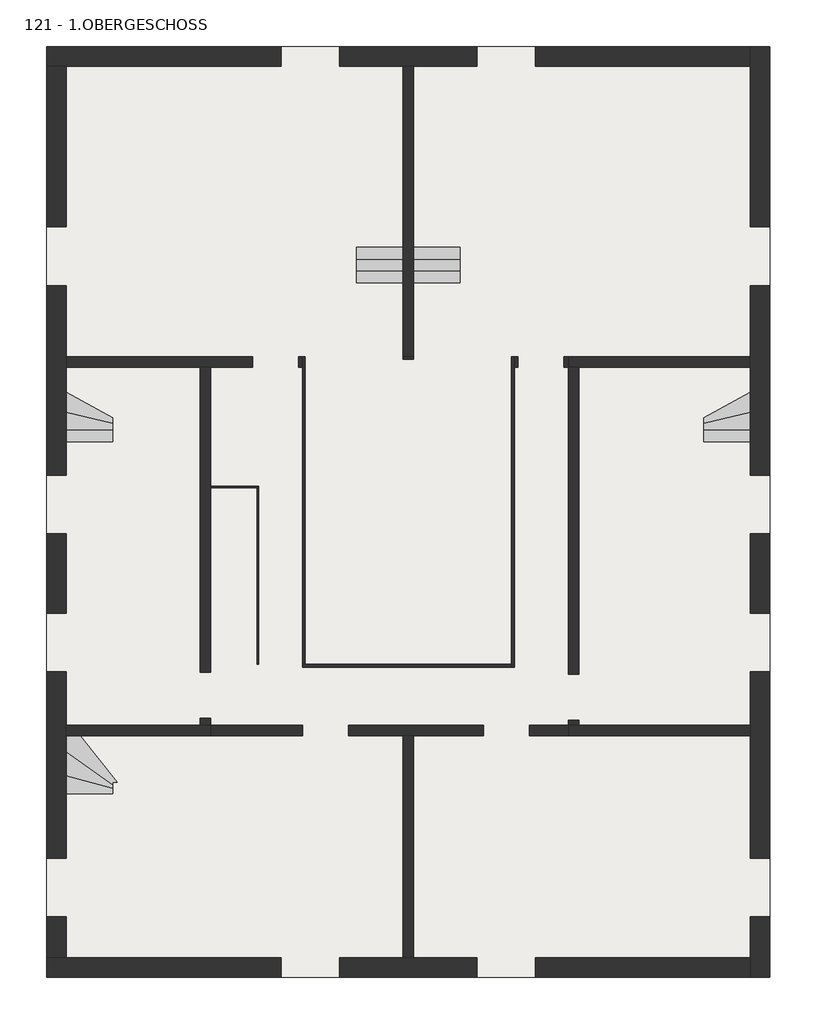
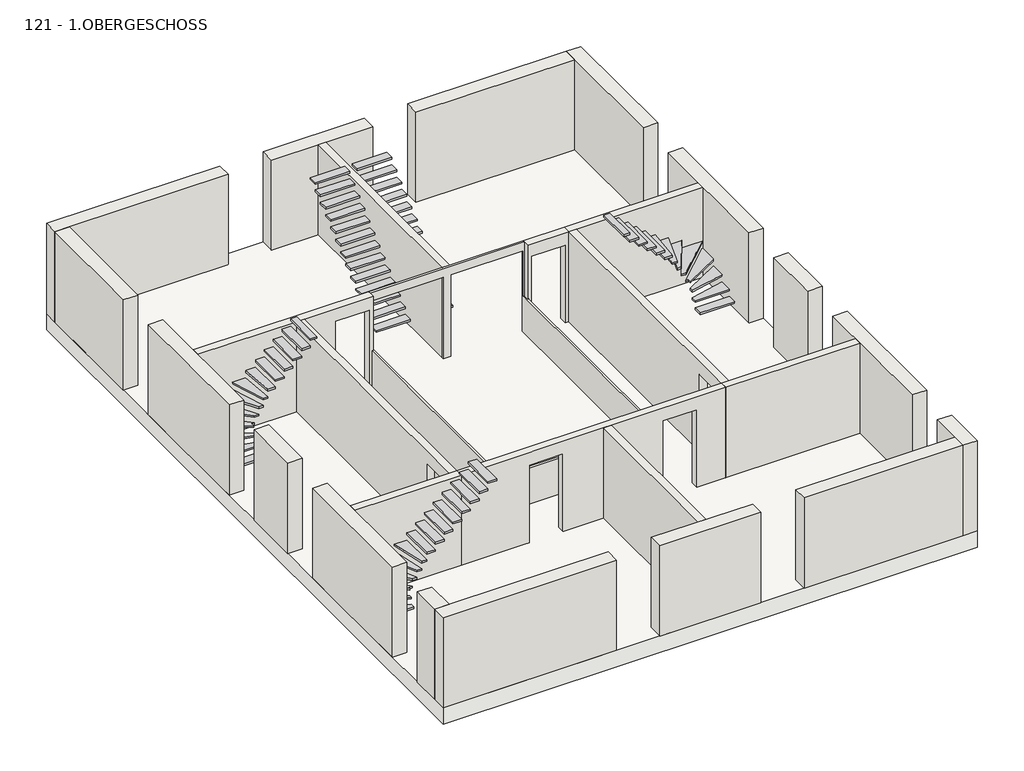
# One storey: 20 walls, 10 stairs, 1 slab.
"""IFC4 building model written with IfcOpenShell, lengths in millimetres."""

import ifcopenshell
import ifcopenshell.guid

model = None  # the IFC model being written
_history = None  # IfcOwnerHistory: only IFC2X3 demands one
_inside = {}  # id of a spatial element -> (the spatial element, [elements in it])
_under = {}  # id of a project, library or spatial element -> (it, [spatial elements below it])
_declared = {}  # id of a project -> (the project, [libraries it declares])
_typed = {}  # id of a type object -> (the type object, [elements of that type])
_made_of = {}  # id of a material, layer set ... -> (it, [elements and type objects made of it])


def new_model(schema):
    """Start an empty IFC model of exactly this schema.

    Asked for "IFC4X3", IfcOpenShell would pick the latest addendum, in which some entities
    have other attributes; the version numbers below select the first issue.
    IFC2X3 requires an IfcOwnerHistory on every rooted entity: one is made here for all.
    """
    global model, _history
    if schema == "IFC4X3":
        model = ifcopenshell.file(schema_version=(4, 3, 0, 0))
    else:
        model = ifcopenshell.file(schema=schema)
    _inside.clear()
    _under.clear()
    _declared.clear()
    _typed.clear()
    _made_of.clear()
    _history = None
    if model.schema == "IFC2X3":
        org = make("IfcOrganization", Name="unknown")
        user = make(
            "IfcPersonAndOrganization",
            ThePerson=make("IfcPerson", FamilyName="unknown"),
            TheOrganization=org,
        )
        app = make(
            "IfcApplication",
            ApplicationDeveloper=org,
            Version="unknown",
            ApplicationFullName="unknown",
            ApplicationIdentifier="unknown",
        )
        _history = make(
            "IfcOwnerHistory",
            OwningUser=user,
            OwningApplication=app,
            ChangeAction="ADDED",
            CreationDate=0,
        )
    return model


def make(cls, **values):
    """One entity of the class cls with the attributes given. An attribute that is None is left unset."""
    return model.create_entity(
        cls, **{name: value for name, value in values.items() if value is not None}
    )


def rooted(cls, **values):
    """An entity with a GlobalId (a new one), such as an element, a storey or a relation."""
    return make(cls, GlobalId=ifcopenshell.guid.new(), OwnerHistory=_history, **values)


def si_unit(unit_type, name, prefix=None):
    """IfcSIUnit, for example si_unit("LENGTHUNIT", "METRE", prefix="MILLI")."""
    return make("IfcSIUnit", UnitType=unit_type, Prefix=prefix, Name=name)


def assignment(units):
    """IfcUnitAssignment: the units of a project."""
    return None if units is None else make("IfcUnitAssignment", Units=units)


def point(xyz):
    """IfcCartesianPoint."""
    return None if xyz is None else make("IfcCartesianPoint", Coordinates=xyz)


def direction(xyz):
    """IfcDirection."""
    return None if xyz is None else make("IfcDirection", DirectionRatios=xyz)


def frame(location, z_axis=None, x_axis=None):
    """IfcAxis2Placement3D, a coordinate frame: its origin and axes. An axis left out is left unset."""
    return make(
        "IfcAxis2Placement3D",
        Location=point(location),
        Axis=direction(z_axis),
        RefDirection=direction(x_axis),
    )


def origin():
    """The frame at (0, 0, 0) with its axes left unset."""
    return frame((0.0, 0.0, 0.0))


def place(relative_to, where):
    """IfcLocalPlacement: puts the frame where relative to a parent placement (None: the world)."""
    return make(
        "IfcLocalPlacement", PlacementRelTo=relative_to, RelativePlacement=where
    )


def context(
    kind, dimensions, precision=None, world=None, true_north=None, identifier=None
):
    """IfcGeometricRepresentationContext, for example the 3D "Model" context."""
    return make(
        "IfcGeometricRepresentationContext",
        ContextIdentifier=identifier,
        ContextType=kind,
        CoordinateSpaceDimension=dimensions,
        Precision=precision,
        WorldCoordinateSystem=world,
        TrueNorth=true_north,
    )


def project(units=None, contexts=None):
    """IfcProject with its units and contexts."""
    return rooted(
        "IfcProject",
        Name="project",
        RepresentationContexts=contexts,
        UnitsInContext=assignment(units),
    )


def spatial(cls, under=None, at=None, **own):
    """A site, building, storey or space (cls), placed at a placement, below another one or the project."""
    s = rooted(cls, ObjectPlacement=at, **own)
    if under is not None:
        _under.setdefault(under.id(), (under, []))[1].append(s)
    return s


def polyline(points):
    """IfcPolyline through the points."""
    return make("IfcPolyline", Points=[point(p) for p in points])


def outline(outer, holes=None, kind="AREA"):
    """IfcArbitraryClosedProfileDef: a profile drawn as a closed curve; with holes, ...WithVoids."""
    if holes is None:
        return make("IfcArbitraryClosedProfileDef", ProfileType=kind, OuterCurve=outer)
    return make(
        "IfcArbitraryProfileDefWithVoids",
        ProfileType=kind,
        OuterCurve=outer,
        InnerCurves=holes,
    )


def extrude(swept, where, along, depth):
    """IfcExtrudedAreaSolid: the profile swept, set in the frame where, extruded along a direction by depth."""
    return make(
        "IfcExtrudedAreaSolid",
        SweptArea=swept,
        Position=where,
        ExtrudedDirection=direction(along),
        Depth=depth,
    )


def faces_of(points, faces, orient=None, outer=None):
    """IfcFace entities. A face is a list of loops; a loop is a list of indices into points, from 0.

    orient and outer hold one flag for each loop. By default every Orientation is true, the
    first loop of a face is its IfcFaceOuterBound and the others are IfcFaceBound.
    """
    made = []
    for i, loops in enumerate(faces):
        bounds = []
        for j, loop in enumerate(loops):
            is_outer = j == 0 if outer is None else outer[i][j]
            bounds.append(
                make(
                    "IfcFaceOuterBound" if is_outer else "IfcFaceBound",
                    Bound=make("IfcPolyLoop", Polygon=[points[k] for k in loop]),
                    Orientation=True if orient is None else orient[i][j],
                )
            )
        made.append(make("IfcFace", Bounds=bounds))
    return made


def faceted_brep(points, faces, orient=None, outer=None, voids=None):
    """IfcFacetedBrep: a solid bounded by flat faces; with voids (closed shells), ...WithVoids."""
    shared = [point(p) for p in points]
    hull = make("IfcClosedShell", CfsFaces=faces_of(shared, faces, orient, outer))
    if voids is None:
        return make("IfcFacetedBrep", Outer=hull)
    return make(
        "IfcFacetedBrepWithVoids",
        Outer=hull,
        Voids=[
            make(cls, CfsFaces=faces_of(shared, fs, o, b)) for cls, fs, o, b in voids
        ],
    )


def shape(context_of_items, identifier, shape_type, items):
    """IfcShapeRepresentation: the items that make up one representation, for example the "Body"."""
    return make(
        "IfcShapeRepresentation",
        ContextOfItems=context_of_items,
        RepresentationIdentifier=identifier,
        RepresentationType=shape_type,
        Items=items,
    )


def source(mapping_origin, context_of_items, identifier, shape_type, items):
    """IfcRepresentationMap: a shape defined once, which mapped items show again and again."""
    return make(
        "IfcRepresentationMap",
        MappingOrigin=mapping_origin,
        MappedRepresentation=shape(context_of_items, identifier, shape_type, items),
    )


def transform(
    local_origin,
    x_axis=None,
    y_axis=None,
    z_axis=None,
    scale=None,
    scale2=None,
    scale3=None,
    uniform=True,
):
    """IfcCartesianTransformationOperator3D, or its non-uniform kind. x_axis, y_axis, z_axis: its Axis1, 2, 3."""
    if uniform:
        return make(
            "IfcCartesianTransformationOperator3D",
            Axis1=direction(x_axis),
            Axis2=direction(y_axis),
            LocalOrigin=point(local_origin),
            Scale=scale,
            Axis3=direction(z_axis),
        )
    return make(
        "IfcCartesianTransformationOperator3DnonUniform",
        Axis1=direction(x_axis),
        Axis2=direction(y_axis),
        LocalOrigin=point(local_origin),
        Scale=scale,
        Axis3=direction(z_axis),
        Scale2=scale2,
        Scale3=scale3,
    )


def mapped(mapping_source, mapping_target):
    """IfcMappedItem: shows the shape of a source again, moved by a transform."""
    return make(
        "IfcMappedItem", MappingSource=mapping_source, MappingTarget=mapping_target
    )


def made_of(thing, what):
    """Note that an element or type object is made of a material, layer set ...; save() writes the relation."""
    if what is not None:
        _made_of.setdefault(what.id(), (what, []))[1].append(thing)
    return thing


def element(
    cls,
    number,
    at=None,
    inside=None,
    cuts=None,
    type_object=None,
    material=None,
    context=None,
    identifier="Body",
    shape_type=None,
    held_by="IfcProductDefinitionShape",
    body=None,
    shapes=None,
    **own,
):
    """One element of the class cls, such as IfcWall. Its Tag is "e" and its number.

    at: its placement. inside: the storey or other place that contains it. cuts: it is an
    opening in that element (IfcRelVoidsElement). A single representation is given by context,
    identifier, shape_type and body (its items); several are given by shapes. held_by: the class
    of the entity that holds the representations. save() writes the other relations.
    """
    e = rooted(cls, Tag="e%d" % number, ObjectPlacement=at, **own)
    if body is not None:
        shapes = [shape(context, identifier, shape_type, body)]
    if shapes is not None:
        e.Representation = make(held_by, Representations=shapes)
    if inside is not None:
        _inside.setdefault(inside.id(), (inside, []))[1].append(e)
    if cuts is not None:
        rooted(
            "IfcRelVoidsElement", RelatingBuildingElement=cuts, RelatedOpeningElement=e
        )
    if type_object is not None:
        _typed.setdefault(type_object.id(), (type_object, []))[1].append(e)
    return made_of(e, material)


def aggregate(whole, parts):
    """IfcRelAggregates: a whole, such as a stair, and the parts it consists of."""
    return rooted("IfcRelAggregates", RelatingObject=whole, RelatedObjects=parts)


def save(model, path):
    """Write the relations noted so far, then the file.

    IfcRelAggregates (storeys below a building ...), IfcRelContainedInSpatialStructure (elements
    in a storey), IfcRelDefinesByType, IfcRelAssociatesMaterial and IfcRelDeclares: one each for
    every whole, place, type object, material and project.
    """
    for whole, parts in _under.values():
        aggregate(whole, parts)
    for where, things in _inside.values():
        rooted(
            "IfcRelContainedInSpatialStructure",
            RelatedElements=things,
            RelatingStructure=where,
        )
    for kind, things in _typed.values():
        rooted("IfcRelDefinesByType", RelatedObjects=things, RelatingType=kind)
    for what, things in _made_of.values():
        rooted("IfcRelAssociatesMaterial", RelatedObjects=things, RelatingMaterial=what)
    for by, libraries in _declared.values():
        rooted("IfcRelDeclares", RelatingContext=by, RelatedDefinitions=libraries)
    model.write(path)


def slab_91406d58(model_context):
    return source(origin(), model_context, "Body", "SweptSolid", [
        extrude(outline(polyline([(15500.0, 19550.0), (15500.0, 1547.1380981), (1500.0, 1547.1380981), (1500.0, 19550.0), (15500.0, 19550.0)])), frame((0.0, 0.0, 2880.0), z_axis=(0.0, 0.0, 1.0), x_axis=(1.0, 0.0, 0.0)), (0.0, 0.0, 1.0), 450.0),
    ])


def stair_92ba3d55(model_context):
    return source(origin(), model_context, "Body", "SweptSolid", [
        extrude(outline(polyline([(160077.7593015, 32139.1812131), (160077.7593015, 32029.7962965), (159177.7593015, 32029.7962965), (159177.7593015, 32381.5903923), (160077.7593015, 32139.1812131)])), frame((0.0, 0.0, 3480.0), z_axis=(0.0, 0.0, 1.0), x_axis=(1.0, 0.0, 0.0)), (0.0, 0.0, 1.0), 50.0),
        extrude(outline(polyline([(160077.7593015, 32208.6851854), (160077.7593015, 32139.1812131), (159177.7593015, 32381.5903923), (159177.7593015, 32851.1265298), (160077.7593015, 32208.6851854)])), frame((0.0, 0.0, 3680.0), z_axis=(0.0, 0.0, 1.0), x_axis=(1.0, 0.0, 0.0)), (0.0, 0.0, 1.0), 50.0),
        extrude(outline(polyline([(159450.38828, 33159.7962965), (160164.4298971, 32259.7962965), (160077.7593015, 32259.7962965), (160077.7593015, 32208.6851854), (159177.7593015, 32851.1265298), (159177.7593015, 33159.7962965), (159450.38828, 33159.7962965)])), frame((0.0, 0.0, 3880.0), z_axis=(0.0, 0.0, 1.0), x_axis=(1.0, 0.0, 0.0)), (0.0, 0.0, 1.0), 50.0),
        extrude(outline(polyline([(160285.4396784, 32259.7962965), (160164.4298971, 32259.7962965), (159450.38828, 33159.7962965), (159877.5404106, 33159.7962965), (160285.4396784, 32259.7962965)])), frame((0.0, 0.0, 4080.0), z_axis=(0.0, 0.0, 1.0), x_axis=(1.0, 0.0, 0.0)), (0.0, 0.0, 1.0), 50.0),
        extrude(outline(polyline([(160412.2916695, 32259.7962965), (160285.4396784, 32259.7962965), (159877.5404106, 33159.7962965), (160212.4306066, 33159.7962965), (160412.2916695, 32259.7962965)])), frame((0.0, 0.0, 4280.0), z_axis=(0.0, 0.0, 1.0), x_axis=(1.0, 0.0, 0.0)), (0.0, 0.0, 1.0), 50.0),
        extrude(outline(polyline([(160546.5910216, 32259.7962965), (160412.2916695, 32259.7962965), (160212.4306066, 33159.7962965), (160538.1312545, 33159.7962965), (160546.5910216, 32259.7962965)])), frame((0.0, 0.0, 4480.0), z_axis=(0.0, 0.0, 1.0), x_axis=(1.0, 0.0, 0.0)), (0.0, 0.0, 1.0), 50.0),
        extrude(outline(polyline([(160772.3611381, 32259.7962965), (160546.5910216, 32259.7962965), (160538.1312545, 33159.7962965), (160772.3611381, 33159.7962965), (160772.3611381, 32259.7962965)])), frame((0.0, 0.0, 4680.0), z_axis=(0.0, 0.0, 1.0), x_axis=(1.0, 0.0, 0.0)), (0.0, 0.0, 1.0), 50.0),
        extrude(outline(polyline([(161002.3611381, 32259.7962965), (160772.3611381, 32259.7962965), (160772.3611381, 33159.7962965), (161002.3611381, 33159.7962965), (161002.3611381, 32259.7962965)])), frame((0.0, 0.0, 4880.0), z_axis=(0.0, 0.0, 1.0), x_axis=(1.0, 0.0, 0.0)), (0.0, 0.0, 1.0), 50.0),
        extrude(outline(polyline([(161232.3611381, 32259.7962965), (161002.3611381, 32259.7962965), (161002.3611381, 33159.7962965), (161232.3611381, 33159.7962965), (161232.3611381, 32259.7962965)])), frame((0.0, 0.0, 5080.0), z_axis=(0.0, 0.0, 1.0), x_axis=(1.0, 0.0, 0.0)), (0.0, 0.0, 1.0), 50.0),
        extrude(outline(polyline([(161462.3611381, 32259.7962965), (161232.3611381, 32259.7962965), (161232.3611381, 33159.7962965), (161462.3611381, 33159.7962965), (161462.3611381, 32259.7962965)])), frame((0.0, 0.0, 5280.0), z_axis=(0.0, 0.0, 1.0), x_axis=(1.0, 0.0, 0.0)), (0.0, 0.0, 1.0), 50.0),
        extrude(outline(polyline([(161692.3611381, 32259.7962965), (161462.3611381, 32259.7962965), (161462.3611381, 33159.7962965), (161692.3611381, 33159.7962965), (161692.3611381, 32259.7962965)])), frame((0.0, 0.0, 5480.0), z_axis=(0.0, 0.0, 1.0), x_axis=(1.0, 0.0, 0.0)), (0.0, 0.0, 1.0), 50.0),
        extrude(outline(polyline([(161922.3611381, 32259.7962965), (161692.3611381, 32259.7962965), (161692.3611381, 33159.7962965), (161922.3611381, 33159.7962965), (161922.3611381, 32259.7962965)])), frame((0.0, 0.0, 5680.0), z_axis=(0.0, 0.0, 1.0), x_axis=(1.0, 0.0, 0.0)), (0.0, 0.0, 1.0), 50.0),
        extrude(outline(polyline([(162152.3611381, 32259.7962965), (161922.3611381, 32259.7962965), (161922.3611381, 33159.7962965), (162152.3611381, 33159.7962965), (162152.3611381, 32259.7962965)])), frame((0.0, 0.0, 5880.0), z_axis=(0.0, 0.0, 1.0), x_axis=(1.0, 0.0, 0.0)), (0.0, 0.0, 1.0), 50.0),
        extrude(outline(polyline([(162382.3611381, 32259.7962965), (162152.3611381, 32259.7962965), (162152.3611381, 33159.7962965), (162382.3611381, 33159.7962965), (162382.3611381, 32259.7962965)])), frame((0.0, 0.0, 6080.0), z_axis=(0.0, 0.0, 1.0), x_axis=(1.0, 0.0, 0.0)), (0.0, 0.0, 1.0), 50.0),
    ])


def stair_5d17669e(model_context):
    return source(origin(), model_context, "Body", "SweptSolid", [
        extrude(outline(polyline([(166797.7593015, 42144.7962965), (166797.7593015, 41914.7962965), (165897.7593015, 41914.7962965), (165897.7593015, 42144.7962965), (166797.7593015, 42144.7962965)])), frame((0.0, 0.0, 3482.1428571), z_axis=(0.0, 0.0, 1.0), x_axis=(1.0, 0.0, 0.0)), (0.0, 0.0, 1.0), 50.0),
        extrude(outline(polyline([(166797.7593015, 42374.7962965), (166797.7593015, 42144.7962965), (165897.7593015, 42144.7962965), (165897.7593015, 42374.7962965), (166797.7593015, 42374.7962965)])), frame((0.0, 0.0, 3684.2857143), z_axis=(0.0, 0.0, 1.0), x_axis=(1.0, 0.0, 0.0)), (0.0, 0.0, 1.0), 50.0),
        extrude(outline(polyline([(166797.7593015, 42604.7962965), (166797.7593015, 42374.7962965), (165897.7593015, 42374.7962965), (165897.7593015, 42604.7962965), (166797.7593015, 42604.7962965)])), frame((0.0, 0.0, 3886.4285714), z_axis=(0.0, 0.0, 1.0), x_axis=(1.0, 0.0, 0.0)), (0.0, 0.0, 1.0), 50.0),
        extrude(outline(polyline([(166797.7593015, 42834.7962965), (166797.7593015, 42604.7962965), (165897.7593015, 42604.7962965), (165897.7593015, 42834.7962965), (166797.7593015, 42834.7962965)])), frame((0.0, 0.0, 4088.5714286), z_axis=(0.0, 0.0, 1.0), x_axis=(1.0, 0.0, 0.0)), (0.0, 0.0, 1.0), 50.0),
        extrude(outline(polyline([(166797.7593015, 43064.7962965), (166797.7593015, 42834.7962965), (165897.7593015, 42834.7962965), (165897.7593015, 43064.7962965), (166797.7593015, 43064.7962965)])), frame((0.0, 0.0, 4290.7142857), z_axis=(0.0, 0.0, 1.0), x_axis=(1.0, 0.0, 0.0)), (0.0, 0.0, 1.0), 50.0),
        extrude(outline(polyline([(166797.7593015, 43294.7962965), (166797.7593015, 43064.7962965), (165897.7593015, 43064.7962965), (165897.7593015, 43294.7962965), (166797.7593015, 43294.7962965)])), frame((0.0, 0.0, 4492.8571429), z_axis=(0.0, 0.0, 1.0), x_axis=(1.0, 0.0, 0.0)), (0.0, 0.0, 1.0), 50.0),
        extrude(outline(polyline([(166797.7593015, 43524.7962965), (166797.7593015, 43294.7962965), (165897.7593015, 43294.7962965), (165897.7593015, 43524.7962965), (166797.7593015, 43524.7962965)])), frame((0.0, 0.0, 4695.0), z_axis=(0.0, 0.0, 1.0), x_axis=(1.0, 0.0, 0.0)), (0.0, 0.0, 1.0), 50.0),
        extrude(outline(polyline([(166797.7593015, 43754.7962965), (166797.7593015, 43524.7962965), (165897.7593015, 43524.7962965), (165897.7593015, 43754.7962965), (166797.7593015, 43754.7962965)])), frame((0.0, 0.0, 4897.1428571), z_axis=(0.0, 0.0, 1.0), x_axis=(1.0, 0.0, 0.0)), (0.0, 0.0, 1.0), 50.0),
        extrude(outline(polyline([(166797.7593015, 43984.7962965), (166797.7593015, 43754.7962965), (165897.7593015, 43754.7962965), (165897.7593015, 43984.7962965), (166797.7593015, 43984.7962965)])), frame((0.0, 0.0, 5099.2857143), z_axis=(0.0, 0.0, 1.0), x_axis=(1.0, 0.0, 0.0)), (0.0, 0.0, 1.0), 50.0),
        extrude(outline(polyline([(166797.7593015, 44214.7962965), (166797.7593015, 43984.7962965), (165897.7593015, 43984.7962965), (165897.7593015, 44214.7962965), (166797.7593015, 44214.7962965)])), frame((0.0, 0.0, 5301.4285714), z_axis=(0.0, 0.0, 1.0), x_axis=(1.0, 0.0, 0.0)), (0.0, 0.0, 1.0), 50.0),
        extrude(outline(polyline([(166797.7593015, 44444.7962965), (166797.7593015, 44214.7962965), (165897.7593015, 44214.7962965), (165897.7593015, 44444.7962965), (166797.7593015, 44444.7962965)])), frame((0.0, 0.0, 5503.5714286), z_axis=(0.0, 0.0, 1.0), x_axis=(1.0, 0.0, 0.0)), (0.0, 0.0, 1.0), 50.0),
        extrude(outline(polyline([(166797.7593015, 44674.7962965), (166797.7593015, 44444.7962965), (165897.7593015, 44444.7962965), (165897.7593015, 44674.7962965), (166797.7593015, 44674.7962965)])), frame((0.0, 0.0, 5705.7142857), z_axis=(0.0, 0.0, 1.0), x_axis=(1.0, 0.0, 0.0)), (0.0, 0.0, 1.0), 50.0),
        extrude(outline(polyline([(166797.7593015, 44904.7962965), (166797.7593015, 44674.7962965), (165897.7593015, 44674.7962965), (165897.7593015, 44904.7962965), (166797.7593015, 44904.7962965)])), frame((0.0, 0.0, 5907.8571429), z_axis=(0.0, 0.0, 1.0), x_axis=(1.0, 0.0, 0.0)), (0.0, 0.0, 1.0), 50.0),
    ])


def stair_42ef58a3(model_context):
    return source(origin(), model_context, "Body", "SweptSolid", [
        extrude(outline(polyline([(165697.7593015, 42144.7962965), (165697.7593015, 41914.7962965), (164797.7593015, 41914.7962965), (164797.7593015, 42144.7962965), (165697.7593015, 42144.7962965)])), frame((0.0, 0.0, 3482.1428571), z_axis=(0.0, 0.0, 1.0), x_axis=(1.0, 0.0, 0.0)), (0.0, 0.0, 1.0), 50.0),
        extrude(outline(polyline([(165697.7593015, 42374.7962965), (165697.7593015, 42144.7962965), (164797.7593015, 42144.7962965), (164797.7593015, 42374.7962965), (165697.7593015, 42374.7962965)])), frame((0.0, 0.0, 3684.2857143), z_axis=(0.0, 0.0, 1.0), x_axis=(1.0, 0.0, 0.0)), (0.0, 0.0, 1.0), 50.0),
        extrude(outline(polyline([(165697.7593015, 42604.7962965), (165697.7593015, 42374.7962965), (164797.7593015, 42374.7962965), (164797.7593015, 42604.7962965), (165697.7593015, 42604.7962965)])), frame((0.0, 0.0, 3886.4285714), z_axis=(0.0, 0.0, 1.0), x_axis=(1.0, 0.0, 0.0)), (0.0, 0.0, 1.0), 50.0),
        extrude(outline(polyline([(165697.7593015, 42834.7962965), (165697.7593015, 42604.7962965), (164797.7593015, 42604.7962965), (164797.7593015, 42834.7962965), (165697.7593015, 42834.7962965)])), frame((0.0, 0.0, 4088.5714286), z_axis=(0.0, 0.0, 1.0), x_axis=(1.0, 0.0, 0.0)), (0.0, 0.0, 1.0), 50.0),
        extrude(outline(polyline([(165697.7593015, 43064.7962965), (165697.7593015, 42834.7962965), (164797.7593015, 42834.7962965), (164797.7593015, 43064.7962965), (165697.7593015, 43064.7962965)])), frame((0.0, 0.0, 4290.7142857), z_axis=(0.0, 0.0, 1.0), x_axis=(1.0, 0.0, 0.0)), (0.0, 0.0, 1.0), 50.0),
        extrude(outline(polyline([(165697.7593015, 43294.7962965), (165697.7593015, 43064.7962965), (164797.7593015, 43064.7962965), (164797.7593015, 43294.7962965), (165697.7593015, 43294.7962965)])), frame((0.0, 0.0, 4492.8571429), z_axis=(0.0, 0.0, 1.0), x_axis=(1.0, 0.0, 0.0)), (0.0, 0.0, 1.0), 50.0),
        extrude(outline(polyline([(165697.7593015, 43524.7962965), (165697.7593015, 43294.7962965), (164797.7593015, 43294.7962965), (164797.7593015, 43524.7962965), (165697.7593015, 43524.7962965)])), frame((0.0, 0.0, 4695.0), z_axis=(0.0, 0.0, 1.0), x_axis=(1.0, 0.0, 0.0)), (0.0, 0.0, 1.0), 50.0),
        extrude(outline(polyline([(165697.7593015, 43754.7962965), (165697.7593015, 43524.7962965), (164797.7593015, 43524.7962965), (164797.7593015, 43754.7962965), (165697.7593015, 43754.7962965)])), frame((0.0, 0.0, 4897.1428571), z_axis=(0.0, 0.0, 1.0), x_axis=(1.0, 0.0, 0.0)), (0.0, 0.0, 1.0), 50.0),
        extrude(outline(polyline([(165697.7593015, 43984.7962965), (165697.7593015, 43754.7962965), (164797.7593015, 43754.7962965), (164797.7593015, 43984.7962965), (165697.7593015, 43984.7962965)])), frame((0.0, 0.0, 5099.2857143), z_axis=(0.0, 0.0, 1.0), x_axis=(1.0, 0.0, 0.0)), (0.0, 0.0, 1.0), 50.0),
        extrude(outline(polyline([(165697.7593015, 44214.7962965), (165697.7593015, 43984.7962965), (164797.7593015, 43984.7962965), (164797.7593015, 44214.7962965), (165697.7593015, 44214.7962965)])), frame((0.0, 0.0, 5301.4285714), z_axis=(0.0, 0.0, 1.0), x_axis=(1.0, 0.0, 0.0)), (0.0, 0.0, 1.0), 50.0),
        extrude(outline(polyline([(165697.7593015, 44444.7962965), (165697.7593015, 44214.7962965), (164797.7593015, 44214.7962965), (164797.7593015, 44444.7962965), (165697.7593015, 44444.7962965)])), frame((0.0, 0.0, 5503.5714286), z_axis=(0.0, 0.0, 1.0), x_axis=(1.0, 0.0, 0.0)), (0.0, 0.0, 1.0), 50.0),
        extrude(outline(polyline([(165697.7593015, 44674.7962965), (165697.7593015, 44444.7962965), (164797.7593015, 44444.7962965), (164797.7593015, 44674.7962965), (165697.7593015, 44674.7962965)])), frame((0.0, 0.0, 5705.7142857), z_axis=(0.0, 0.0, 1.0), x_axis=(1.0, 0.0, 0.0)), (0.0, 0.0, 1.0), 50.0),
        extrude(outline(polyline([(165697.7593015, 44904.7962965), (165697.7593015, 44674.7962965), (164797.7593015, 44674.7962965), (164797.7593015, 44904.7962965), (165697.7593015, 44904.7962965)])), frame((0.0, 0.0, 5907.8571429), z_axis=(0.0, 0.0, 1.0), x_axis=(1.0, 0.0, 0.0)), (0.0, 0.0, 1.0), 50.0),
    ])


def stair_4856ba97(model_context):
    return source(origin(), model_context, "Body", "SweptSolid", [
        extrude(outline(polyline([(159177.7593015, 39074.7962965), (160077.7593015, 39074.7962965), (160077.7593015, 38844.7962965), (159177.7593015, 38844.7962965), (159177.7593015, 39074.7962965)])), frame((0.0, 0.0, 3482.1428571), z_axis=(0.0, 0.0, 1.0), x_axis=(1.0, 0.0, 0.0)), (0.0, 0.0, 1.0), 50.0),
        extrude(outline(polyline([(159177.7593015, 39407.7634868), (160077.7593015, 39201.8291061), (160077.7593015, 39074.7962965), (159177.7593015, 39074.7962965), (159177.7593015, 39407.7634868)])), frame((0.0, 0.0, 3684.2857143), z_axis=(0.0, 0.0, 1.0), x_axis=(1.0, 0.0, 0.0)), (0.0, 0.0, 1.0), 50.0),
        extrude(outline(polyline([(159177.7593015, 39801.0914939), (160077.7593015, 39301.7193734), (160077.7593015, 39201.8291061), (159177.7593015, 39407.7634868), (159177.7593015, 39801.0914939)])), frame((0.0, 0.0, 3886.4285714), z_axis=(0.0, 0.0, 1.0), x_axis=(1.0, 0.0, 0.0)), (0.0, 0.0, 1.0), 50.0),
        extrude(outline(polyline([(159177.7593015, 40284.7962965), (159200.4297176, 40284.7962965), (160147.7593015, 39384.7962965), (160077.7593015, 39384.7962965), (160077.7593015, 39301.7193734), (159177.7593015, 39801.0914939), (159177.7593015, 40284.7962965)])), frame((0.0, 0.0, 4088.5714286), z_axis=(0.0, 0.0, 1.0), x_axis=(1.0, 0.0, 0.0)), (0.0, 0.0, 1.0), 50.0),
        extrude(outline(polyline([(159730.1980238, 40284.7962965), (160258.7713888, 39384.7962965), (160147.7593015, 39384.7962965), (159200.4297176, 40284.7962965), (159730.1980238, 40284.7962965)])), frame((0.0, 0.0, 4290.7142857), z_axis=(0.0, 0.0, 1.0), x_axis=(1.0, 0.0, 0.0)), (0.0, 0.0, 1.0), 50.0),
        extrude(outline(polyline([(160089.4284981, 40284.7962965), (160375.293778, 39384.7962965), (160258.7713888, 39384.7962965), (159730.1980238, 40284.7962965), (160089.4284981, 40284.7962965)])), frame((0.0, 0.0, 4492.8571429), z_axis=(0.0, 0.0, 1.0), x_axis=(1.0, 0.0, 0.0)), (0.0, 0.0, 1.0), 50.0),
        extrude(outline(polyline([(160425.6183342, 40284.7962965), (160499.1039419, 39384.7962965), (160375.293778, 39384.7962965), (160089.4284981, 40284.7962965), (160425.6183342, 40284.7962965)])), frame((0.0, 0.0, 4695.0), z_axis=(0.0, 0.0, 1.0), x_axis=(1.0, 0.0, 0.0)), (0.0, 0.0, 1.0), 50.0),
        extrude(outline(polyline([(160692.3611381, 40284.7962965), (160692.3611381, 39384.7962965), (160499.1039419, 39384.7962965), (160425.6183342, 40284.7962965), (160692.3611381, 40284.7962965)])), frame((0.0, 0.0, 4897.1428571), z_axis=(0.0, 0.0, 1.0), x_axis=(1.0, 0.0, 0.0)), (0.0, 0.0, 1.0), 50.0),
        extrude(outline(polyline([(160922.3611381, 40284.7962965), (160922.3611381, 39384.7962965), (160692.3611381, 39384.7962965), (160692.3611381, 40284.7962965), (160922.3611381, 40284.7962965)])), frame((0.0, 0.0, 5099.2857143), z_axis=(0.0, 0.0, 1.0), x_axis=(1.0, 0.0, 0.0)), (0.0, 0.0, 1.0), 50.0),
        extrude(outline(polyline([(161152.3611381, 40284.7962965), (161152.3611381, 39384.7962965), (160922.3611381, 39384.7962965), (160922.3611381, 40284.7962965), (161152.3611381, 40284.7962965)])), frame((0.0, 0.0, 5301.4285714), z_axis=(0.0, 0.0, 1.0), x_axis=(1.0, 0.0, 0.0)), (0.0, 0.0, 1.0), 50.0),
        extrude(outline(polyline([(161382.3611381, 40284.7962965), (161382.3611381, 39384.7962965), (161152.3611381, 39384.7962965), (161152.3611381, 40284.7962965), (161382.3611381, 40284.7962965)])), frame((0.0, 0.0, 5503.5714286), z_axis=(0.0, 0.0, 1.0), x_axis=(1.0, 0.0, 0.0)), (0.0, 0.0, 1.0), 50.0),
        extrude(outline(polyline([(161612.3611381, 40284.7962965), (161612.3611381, 39384.7962965), (161382.3611381, 39384.7962965), (161382.3611381, 40284.7962965), (161612.3611381, 40284.7962965)])), frame((0.0, 0.0, 5705.7142857), z_axis=(0.0, 0.0, 1.0), x_axis=(1.0, 0.0, 0.0)), (0.0, 0.0, 1.0), 50.0),
        extrude(outline(polyline([(161772.7593015, 40284.7962965), (161772.7593015, 39384.7962965), (161612.3611381, 39384.7962965), (161612.3611381, 40284.7962965), (161772.7593015, 40284.7962965)])), frame((0.0, 0.0, 5907.8571429), z_axis=(0.0, 0.0, 1.0), x_axis=(1.0, 0.0, 0.0)), (0.0, 0.0, 1.0), 50.0),
    ])


def stair_6893023c(model_context):
    return source(origin(), model_context, "Body", "SweptSolid", [
        extrude(outline(polyline([(171517.7593015, 39074.7962965), (172417.7593015, 39074.7962965), (172417.7593015, 38844.7962965), (171517.7593015, 38844.7962965), (171517.7593015, 39074.7962965)])), frame((0.0, 0.0, 3482.1428571), z_axis=(0.0, 0.0, 1.0), x_axis=(1.0, 0.0, 0.0)), (0.0, 0.0, 1.0), 50.0),
        extrude(outline(polyline([(171517.7593015, 39201.8291061), (172417.7593015, 39407.7634868), (172417.7593015, 39074.7962965), (171517.7593015, 39074.7962965), (171517.7593015, 39201.8291061)])), frame((0.0, 0.0, 3684.2857143), z_axis=(0.0, 0.0, 1.0), x_axis=(1.0, 0.0, 0.0)), (0.0, 0.0, 1.0), 50.0),
        extrude(outline(polyline([(171517.7593015, 39301.7193734), (172417.7593015, 39801.0914939), (172417.7593015, 39407.7634868), (171517.7593015, 39201.8291061), (171517.7593015, 39301.7193734)])), frame((0.0, 0.0, 3886.4285714), z_axis=(0.0, 0.0, 1.0), x_axis=(1.0, 0.0, 0.0)), (0.0, 0.0, 1.0), 50.0),
        extrude(outline(polyline([(171517.7593015, 39384.7962965), (171447.7593015, 39384.7962965), (172395.0888853, 40284.7962965), (172417.7593015, 40284.7962965), (172417.7593015, 39801.0914939), (171517.7593015, 39301.7193734), (171517.7593015, 39384.7962965)])), frame((0.0, 0.0, 4088.5714286), z_axis=(0.0, 0.0, 1.0), x_axis=(1.0, 0.0, 0.0)), (0.0, 0.0, 1.0), 50.0),
        extrude(outline(polyline([(171336.7472141, 39384.7962965), (171865.3205791, 40284.7962965), (172395.0888853, 40284.7962965), (171447.7593015, 39384.7962965), (171336.7472141, 39384.7962965)])), frame((0.0, 0.0, 4290.7142857), z_axis=(0.0, 0.0, 1.0), x_axis=(1.0, 0.0, 0.0)), (0.0, 0.0, 1.0), 50.0),
        extrude(outline(polyline([(171220.2248249, 39384.7962965), (171506.0901048, 40284.7962965), (171865.3205791, 40284.7962965), (171336.7472141, 39384.7962965), (171220.2248249, 39384.7962965)])), frame((0.0, 0.0, 4492.8571429), z_axis=(0.0, 0.0, 1.0), x_axis=(1.0, 0.0, 0.0)), (0.0, 0.0, 1.0), 50.0),
        extrude(outline(polyline([(171096.414661, 39384.7962965), (171169.9002687, 40284.7962965), (171506.0901048, 40284.7962965), (171220.2248249, 39384.7962965), (171096.414661, 39384.7962965)])), frame((0.0, 0.0, 4695.0), z_axis=(0.0, 0.0, 1.0), x_axis=(1.0, 0.0, 0.0)), (0.0, 0.0, 1.0), 50.0),
        extrude(outline(polyline([(170903.1574649, 39384.7962965), (170903.1574649, 40284.7962965), (171169.9002687, 40284.7962965), (171096.414661, 39384.7962965), (170903.1574649, 39384.7962965)])), frame((0.0, 0.0, 4897.1428571), z_axis=(0.0, 0.0, 1.0), x_axis=(1.0, 0.0, 0.0)), (0.0, 0.0, 1.0), 50.0),
        extrude(outline(polyline([(170673.1574649, 39384.7962965), (170673.1574649, 40284.7962965), (170903.1574649, 40284.7962965), (170903.1574649, 39384.7962965), (170673.1574649, 39384.7962965)])), frame((0.0, 0.0, 5099.2857143), z_axis=(0.0, 0.0, 1.0), x_axis=(1.0, 0.0, 0.0)), (0.0, 0.0, 1.0), 50.0),
        extrude(outline(polyline([(170443.1574649, 39384.7962965), (170443.1574649, 40284.7962965), (170673.1574649, 40284.7962965), (170673.1574649, 39384.7962965), (170443.1574649, 39384.7962965)])), frame((0.0, 0.0, 5301.4285714), z_axis=(0.0, 0.0, 1.0), x_axis=(1.0, 0.0, 0.0)), (0.0, 0.0, 1.0), 50.0),
        extrude(outline(polyline([(170213.1574649, 39384.7962965), (170213.1574649, 40284.7962965), (170443.1574649, 40284.7962965), (170443.1574649, 39384.7962965), (170213.1574649, 39384.7962965)])), frame((0.0, 0.0, 5503.5714286), z_axis=(0.0, 0.0, 1.0), x_axis=(1.0, 0.0, 0.0)), (0.0, 0.0, 1.0), 50.0),
        extrude(outline(polyline([(169983.1574649, 39384.7962965), (169983.1574649, 40284.7962965), (170213.1574649, 40284.7962965), (170213.1574649, 39384.7962965), (169983.1574649, 39384.7962965)])), frame((0.0, 0.0, 5705.7142857), z_axis=(0.0, 0.0, 1.0), x_axis=(1.0, 0.0, 0.0)), (0.0, 0.0, 1.0), 50.0),
        extrude(outline(polyline([(169822.7593015, 39384.7962965), (169822.7593015, 40284.7962965), (169983.1574649, 40284.7962965), (169983.1574649, 39384.7962965), (169822.7593015, 39384.7962965)])), frame((0.0, 0.0, 5907.8571429), z_axis=(0.0, 0.0, 1.0), x_axis=(1.0, 0.0, 0.0)), (0.0, 0.0, 1.0), 50.0),
    ])


model = new_model("IFC4")

# Units and contexts
model_context = context("Model", 3, world=origin())
ifc_project = project(units=[si_unit("LENGTHUNIT", "METRE", prefix="MILLI")], contexts=[model_context])

# Site, building, storey
site = spatial("IfcSite", under=ifc_project)
building = spatial("IfcBuilding", under=site)
storey = spatial("IfcBuildingStorey", under=building, Name="121 - 1.OBERGESCHOSS", Elevation=2825.0)

# Slab
placement = place(None, origin())
slab_shape = slab_91406d58(model_context)
element("IfcSlab", 1, ObjectType="Holzdecke 176 : Holzdecke 176", at=placement, inside=storey, context=model_context, shape_type="MappedRepresentation", body=[
    mapped(slab_shape, transform((0.0, 0.0, 0.0), x_axis=(1.0, 0.0, 0.0), y_axis=(0.0, 1.0, 0.0), z_axis=(0.0, 0.0, 1.0))),
])

# Stairs
stair_shape = stair_92ba3d55(model_context)
element("IfcStair", 2, ObjectType="  97010 :   97010", at=placement, inside=storey, context=model_context, shape_type="MappedRepresentation", body=[
    mapped(stair_shape, transform((-157297.7593015, -26934.7962965, 0.0), x_axis=(1.0, 0.0, 0.0), y_axis=(0.0, 1.0, 0.0), z_axis=(0.0, 0.0, 1.0))),
])
stair_2_shape = stair_5d17669e(model_context)
element("IfcStair", 3, ObjectType="  97882 :   97882", at=placement, inside=storey, context=model_context, shape_type="MappedRepresentation", body=[
    mapped(stair_2_shape, transform((-157297.7593015, -26934.7962965, 0.0), x_axis=(1.0, 0.0, 0.0), y_axis=(0.0, 1.0, 0.0), z_axis=(0.0, 0.0, 1.0))),
])
stair_3_shape = stair_42ef58a3(model_context)
element("IfcStair", 4, ObjectType="  98300 :   98300", at=placement, inside=storey, context=model_context, shape_type="MappedRepresentation", body=[
    mapped(stair_3_shape, transform((-157297.7593015, -26934.7962965, 0.0), x_axis=(1.0, 0.0, 0.0), y_axis=(0.0, 1.0, 0.0), z_axis=(0.0, 0.0, 1.0))),
])
stair_4_shape = stair_4856ba97(model_context)
element("IfcStair", 5, ObjectType="  98728 :   98728", at=placement, inside=storey, context=model_context, shape_type="MappedRepresentation", body=[
    mapped(stair_4_shape, transform((-157297.7593015, -26934.7962965, 0.0), x_axis=(1.0, 0.0, 0.0), y_axis=(0.0, 1.0, 0.0), z_axis=(0.0, 0.0, 1.0))),
])
stair_5_shape = stair_6893023c(model_context)
element("IfcStair", 6, ObjectType="  99154 :   99154", at=placement, inside=storey, context=model_context, shape_type="MappedRepresentation", body=[
    mapped(stair_5_shape, transform((-157297.7593015, -26934.7962965, 0.0), x_axis=(1.0, 0.0, 0.0), y_axis=(0.0, 1.0, 0.0), z_axis=(0.0, 0.0, 1.0))),
])
element("IfcStair", 7, ObjectType="  149542 :   149542", at=placement, inside=storey, context=model_context, shape_type="MappedRepresentation", body=[
    mapped(stair_shape, transform((-157297.7593015, -26934.7962965, 0.0), x_axis=(1.0, 0.0, 0.0), y_axis=(0.0, 1.0, 0.0), z_axis=(0.0, 0.0, 1.0))),
])
element("IfcStair", 8, ObjectType="  150414 :   150414", at=placement, inside=storey, context=model_context, shape_type="MappedRepresentation", body=[
    mapped(stair_2_shape, transform((-157297.7593015, -26934.7962965, 0.0), x_axis=(1.0, 0.0, 0.0), y_axis=(0.0, 1.0, 0.0), z_axis=(0.0, 0.0, 1.0))),
])
element("IfcStair", 9, ObjectType="  150832 :   150832", at=placement, inside=storey, context=model_context, shape_type="MappedRepresentation", body=[
    mapped(stair_3_shape, transform((-157297.7593015, -26934.7962965, 0.0), x_axis=(1.0, 0.0, 0.0), y_axis=(0.0, 1.0, 0.0), z_axis=(0.0, 0.0, 1.0))),
])
element("IfcStair", 10, ObjectType="  151260 :   151260", at=placement, inside=storey, context=model_context, shape_type="MappedRepresentation", body=[
    mapped(stair_4_shape, transform((-157297.7593015, -26934.7962965, 0.0), x_axis=(1.0, 0.0, 0.0), y_axis=(0.0, 1.0, 0.0), z_axis=(0.0, 0.0, 1.0))),
])
element("IfcStair", 11, ObjectType="  151686 :   151686", at=placement, inside=storey, context=model_context, shape_type="MappedRepresentation", body=[
    mapped(stair_5_shape, transform((-157297.7593015, -26934.7962965, 0.0), x_axis=(1.0, 0.0, 0.0), y_axis=(0.0, 1.0, 0.0), z_axis=(0.0, 0.0, 1.0))),
])

# Walls
element("IfcWall", 12, ObjectType=" :1152", at=placement, inside=storey, context=model_context, shape_type="Brep", body=[
    faceted_brep([(15120.0, 14926.9335014, 5830.0), (15120.0, 14926.9335014, 3330.0), (15120.0, 11259.602585, 3330.0), (15120.0, 11259.602585, 5830.0), (15500.0, 14926.9335014, 3330.0), (15500.0, 14926.9335014, 5830.0), (15500.0, 11259.602585, 5830.0), (15500.0, 11259.602585, 3330.0)], [[[0, 1, 2, 3]], [[4, 5, 6, 7]], [[1, 4, 7, 2]], [[5, 0, 3, 6]], [[1, 0, 5, 4]], [[3, 2, 7, 6]]]),
    faceted_brep([(15120.0, 10124.602585, 5830.0), (15120.0, 10124.602585, 3330.0), (15120.0, 8593.5588642, 3330.0), (15120.0, 8593.5588642, 5830.0), (15500.0, 10124.602585, 3330.0), (15500.0, 10124.602585, 5830.0), (15500.0, 8593.5588642, 5830.0), (15500.0, 8593.5588642, 3330.0)], [[[0, 1, 2, 3]], [[4, 5, 6, 7]], [[1, 4, 7, 2]], [[5, 0, 3, 6]], [[1, 0, 5, 4]], [[3, 2, 7, 6]]]),
    faceted_brep([(15120.0, 7458.5588642, 5830.0), (15120.0, 7458.5588642, 3330.0), (15120.0, 3851.740683, 3330.0), (15120.0, 3851.740683, 5830.0), (15500.0, 7458.5588642, 3330.0), (15500.0, 7458.5588642, 5830.0), (15500.0, 3851.740683, 5830.0), (15500.0, 3851.740683, 3330.0)], [[[0, 1, 2, 3]], [[4, 5, 6, 7]], [[1, 4, 7, 2]], [[5, 0, 3, 6]], [[1, 0, 5, 4]], [[3, 2, 7, 6]]]),
    faceted_brep([(15120.0, 19550.0, 3330.0), (15120.0, 19170.0, 3330.0), (15120.0, 16061.9335014, 3330.0), (15120.0, 16061.9335014, 5830.0), (15120.0, 19170.0, 5830.0), (15120.0, 19550.0, 5830.0), (15500.0, 19550.0, 5830.0), (15500.0, 16061.9335014, 5830.0), (15500.0, 16061.9335014, 3330.0), (15500.0, 19550.0, 3330.0)], [[[0, 1, 2, 3, 4, 5]], [[6, 7, 8, 9]], [[2, 1, 0, 9, 8]], [[5, 4, 3, 7, 6]], [[3, 2, 8, 7]], [[0, 5, 6, 9]]]),
    faceted_brep([(15120.0, 1547.1380981, 3330.0), (15120.0, 1547.1380981, 5830.0), (15120.0, 1927.1380981, 5830.0), (15120.0, 2716.740683, 5830.0), (15120.0, 2716.740683, 3330.0), (15120.0, 1927.1380981, 3330.0), (15500.0, 1547.1380981, 5830.0), (15500.0, 1547.1380981, 3330.0), (15500.0, 2716.740683, 3330.0), (15500.0, 2716.740683, 5830.0)], [[[0, 1, 2, 3, 4, 5]], [[6, 7, 8, 9]], [[7, 0, 5, 4, 8]], [[1, 6, 9, 3, 2]], [[4, 3, 9, 8]], [[1, 0, 7, 6]]]),
])
element("IfcWall", 13, ObjectType=" :1161", at=placement, inside=storey, context=model_context, shape_type="Brep", body=[
    faceted_brep([(15120.0, 1927.1380981, 3330.0), (10960.0, 1927.1380981, 3330.0), (10960.0, 1927.1380981, 5830.0), (15120.0, 1927.1380981, 5830.0), (15120.0, 1547.1380981, 5830.0), (10960.0, 1547.1380981, 5830.0), (10960.0, 1547.1380981, 3330.0), (15120.0, 1547.1380981, 3330.0)], [[[0, 1, 2, 3]], [[4, 5, 6, 7]], [[1, 0, 7, 6]], [[3, 2, 5, 4]], [[2, 1, 6, 5]], [[0, 3, 4, 7]]]),
    faceted_brep([(9825.0, 1927.1380981, 5830.0), (9825.0, 1927.1380981, 3330.0), (7175.0, 1927.1380981, 3330.0), (7175.0, 1927.1380981, 5830.0), (9825.0, 1547.1380981, 3330.0), (9825.0, 1547.1380981, 5830.0), (7175.0, 1547.1380981, 5830.0), (7175.0, 1547.1380981, 3330.0)], [[[0, 1, 2, 3]], [[4, 5, 6, 7]], [[1, 4, 7, 2]], [[5, 0, 3, 6]], [[1, 0, 5, 4]], [[3, 2, 7, 6]]]),
    faceted_brep([(1500.0, 1927.1380981, 3330.0), (1500.0, 1927.1380981, 5830.0), (1880.0, 1927.1380981, 5830.0), (6040.0, 1927.1380981, 5830.0), (6040.0, 1927.1380981, 3330.0), (1880.0, 1927.1380981, 3330.0), (1500.0, 1547.1380981, 5830.0), (1500.0, 1547.1380981, 3330.0), (6040.0, 1547.1380981, 3330.0), (6040.0, 1547.1380981, 5830.0)], [[[0, 1, 2, 3, 4, 5]], [[6, 7, 8, 9]], [[7, 0, 5, 4, 8]], [[1, 6, 9, 3, 2]], [[4, 3, 9, 8]], [[1, 0, 7, 6]]]),
])
element("IfcWall", 14, ObjectType=" :1164", at=placement, inside=storey, context=model_context, shape_type="Brep", body=[
    faceted_brep([(10960.0, 19170.0, 3330.0), (15120.0, 19170.0, 3330.0), (15120.0, 19170.0, 5830.0), (10960.0, 19170.0, 5830.0), (10960.0, 19550.0, 5830.0), (15120.0, 19550.0, 5830.0), (15120.0, 19550.0, 3330.0), (10960.0, 19550.0, 3330.0)], [[[0, 1, 2, 3]], [[4, 5, 6, 7]], [[1, 0, 7, 6]], [[3, 2, 5, 4]], [[0, 3, 4, 7]], [[2, 1, 6, 5]]]),
    faceted_brep([(9825.0, 19170.0, 3330.0), (9825.0, 19170.0, 5830.0), (7175.0, 19170.0, 5830.0), (7175.0, 19170.0, 3330.0), (9825.0, 19550.0, 5830.0), (9825.0, 19550.0, 3330.0), (7175.0, 19550.0, 3330.0), (7175.0, 19550.0, 5830.0)], [[[0, 1, 2, 3]], [[4, 5, 6, 7]], [[5, 0, 3, 6]], [[1, 4, 7, 2]], [[1, 0, 5, 4]], [[3, 2, 7, 6]]]),
    faceted_brep([(1500.0, 19170.0, 5830.0), (1500.0, 19170.0, 3330.0), (1880.0, 19170.0, 3330.0), (6040.0, 19170.0, 3330.0), (6040.0, 19170.0, 5830.0), (1880.0, 19170.0, 5830.0), (1500.0, 19550.0, 3330.0), (1500.0, 19550.0, 5830.0), (6040.0, 19550.0, 5830.0), (6040.0, 19550.0, 3330.0)], [[[0, 1, 2, 3, 4, 5]], [[6, 7, 8, 9]], [[1, 6, 9, 3, 2]], [[7, 0, 5, 4, 8]], [[4, 3, 9, 8]], [[1, 0, 7, 6]]]),
])
element("IfcWall", 15, ObjectType=" :1165", at=placement, inside=storey, context=model_context, shape_type="SweptSolid", body=[
    extrude(outline(polyline([(1880.0, 19170.0), (1880.0, 16061.9335014), (1500.0, 16061.9335014), (1500.0, 19170.0), (1880.0, 19170.0)])), frame((0.0, 0.0, 3330.0), z_axis=(0.0, 0.0, 1.0), x_axis=(1.0, 0.0, 0.0)), (0.0, 0.0, 1.0), 2500.0),
    extrude(outline(polyline([(1500.0, 14926.9335014), (1880.0, 14926.9335014), (1880.0, 11259.602585), (1500.0, 11259.602585), (1500.0, 14926.9335014)])), frame((0.0, 0.0, 3330.0), z_axis=(0.0, 0.0, 1.0), x_axis=(1.0, 0.0, 0.0)), (0.0, 0.0, 1.0), 2500.0),
    extrude(outline(polyline([(1500.0, 10124.602585), (1880.0, 10124.602585), (1880.0, 8593.5588642), (1500.0, 8593.5588642), (1500.0, 10124.602585)])), frame((0.0, 0.0, 3330.0), z_axis=(0.0, 0.0, 1.0), x_axis=(1.0, 0.0, 0.0)), (0.0, 0.0, 1.0), 2500.0),
    extrude(outline(polyline([(1500.0, 7458.5588642), (1880.0, 7458.5588642), (1880.0, 3851.740683), (1500.0, 3851.740683), (1500.0, 7458.5588642)])), frame((0.0, 0.0, 3330.0), z_axis=(0.0, 0.0, 1.0), x_axis=(1.0, 0.0, 0.0)), (0.0, 0.0, 1.0), 2500.0),
    extrude(outline(polyline([(1880.0, 1927.1380981), (1500.0, 1927.1380981), (1500.0, 2716.740683), (1880.0, 2716.740683), (1880.0, 1927.1380981)])), frame((0.0, 0.0, 3330.0), z_axis=(0.0, 0.0, 1.0), x_axis=(1.0, 0.0, 0.0)), (0.0, 0.0, 1.0), 2500.0),
])
element("IfcWall", 16, ObjectType=" :1166", at=placement, inside=storey, context=model_context, shape_type="SweptSolid", body=[
    extrude(outline(polyline([(5830.0, 10525.0), (5830.0, 6475.0), (4330.0, 6475.0), (4330.0, 6500.0), (5590.0, 6500.0), (5590.0, 8400.0), (3330.0, 8400.0), (3330.0, 8600.0), (5590.0, 8600.0), (5590.0, 10500.0), (4330.0, 10500.0), (4330.0, 10525.0), (5830.0, 10525.0)])), frame((0.0, 13500.0, 0.0), z_axis=(0.0, 1.0, 0.0), x_axis=(0.0, 0.0, 1.0)), (0.0, 0.0, 1.0), 50.0),
])
element("IfcWall", 17, ObjectType="Holzwand:1150", at=placement, inside=storey, context=model_context, shape_type="Brep", body=[
    faceted_brep([(11600.0, 13350.0, 3330.0), (11800.0, 13350.0, 3330.0), (15120.0, 13350.0, 3330.0), (15120.0, 13350.0, 5830.0), (11800.0, 13350.0, 5830.0), (11600.0, 13350.0, 5830.0), (11600.0, 13550.0, 3330.0), (11600.0, 13550.0, 5830.0), (15120.0, 13550.0, 5830.0), (15120.0, 13550.0, 3330.0)], [[[0, 1, 2, 3, 4, 5]], [[6, 7, 8, 9]], [[2, 1, 0, 6, 9]], [[5, 4, 3, 8, 7]], [[0, 5, 7, 6]], [[3, 2, 9, 8]]]),
])
element("IfcWall", 18, ObjectType="Holzwand:1151", at=placement, inside=storey, context=model_context, shape_type="Brep", body=[
    faceted_brep([(4675.0, 6425.0, 3330.0), (4475.0, 6425.0, 3330.0), (1880.0, 6425.0, 3330.0), (1880.0, 6425.0, 5830.0), (4475.0, 6425.0, 5830.0), (4675.0, 6425.0, 5830.0), (4675.0, 6225.0, 3330.0), (4675.0, 6225.0, 5830.0), (1880.0, 6225.0, 5830.0), (1880.0, 6225.0, 3330.0)], [[[0, 1, 2, 3, 4, 5]], [[6, 7, 8, 9]], [[2, 1, 0, 6, 9]], [[5, 4, 3, 8, 7]], [[0, 5, 7, 6]], [[3, 2, 9, 8]]]),
])
element("IfcWall", 19, ObjectType="Holzwand:1153", at=placement, inside=storey, context=model_context, shape_type="Brep", body=[
    faceted_brep([(15120.0, 6425.0, 3330.0), (11800.0, 6425.0, 3330.0), (11600.0, 6425.0, 3330.0), (11600.0, 6425.0, 5830.0), (11800.0, 6425.0, 5830.0), (15120.0, 6425.0, 5830.0), (15120.0, 6225.0, 3330.0), (15120.0, 6225.0, 5830.0), (11600.0, 6225.0, 5830.0), (11600.0, 6225.0, 3330.0)], [[[0, 1, 2, 3, 4, 5]], [[6, 7, 8, 9]], [[2, 1, 0, 6, 9]], [[5, 4, 3, 8, 7]], [[3, 2, 9, 8]], [[0, 5, 7, 6]]]),
])
element("IfcWall", 20, ObjectType="Holzwand:1154", at=placement, inside=storey, context=model_context, shape_type="Brep", body=[
    faceted_brep([(5605.0, 11050.0, 3330.0), (4675.0, 11050.0, 3330.0), (4675.0, 11050.0, 4330.0), (5605.0, 11050.0, 4330.0), (5605.0, 11020.0, 3330.0), (5605.0, 11020.0, 4330.0), (5575.0, 11020.0, 4330.0), (4675.0, 11020.0, 4330.0), (4675.0, 11020.0, 3330.0), (5575.0, 11020.0, 3330.0)], [[[0, 1, 2, 3]], [[4, 5, 6, 7, 8, 9]], [[1, 0, 4, 9, 8]], [[3, 2, 7, 6, 5]], [[0, 3, 5, 4]], [[2, 1, 8, 7]]]),
])
element("IfcWall", 21, ObjectType="Holzwand:1155", at=placement, inside=storey, context=model_context, shape_type="SweptSolid", body=[
    extrude(outline(polyline([(5605.0, 11020.0), (5605.0, 7600.0), (5575.0, 7600.0), (5575.0, 11020.0), (5605.0, 11020.0)])), frame((0.0, 0.0, 3330.0), z_axis=(0.0, 0.0, 1.0), x_axis=(1.0, 0.0, 0.0)), (0.0, 0.0, 1.0), 1000.0),
])
element("IfcWall", 22, ObjectType="Holzwand:1156", at=placement, inside=storey, context=model_context, shape_type="SweptSolid", body=[
    extrude(outline(polyline([(6425.0, 5830.0), (13350.0, 5830.0), (13350.0, 3330.0), (7409.5766702, 3330.0), (7409.5766702, 5480.0), (6524.5766702, 5480.0), (6524.5766702, 3330.0), (6425.0, 3330.0), (6425.0, 5830.0)])), frame((11600.0, 0.0, 0.0), z_axis=(1.0, 0.0, 0.0), x_axis=(0.0, 1.0, 0.0)), (0.0, 0.0, 1.0), 200.0),
])
element("IfcWall", 23, ObjectType="Holzwand:1157", at=placement, inside=storey, context=model_context, shape_type="SweptSolid", body=[
    extrude(outline(polyline([(8600.0, 19170.0), (8600.0, 13550.0), (8400.0, 13550.0), (8400.0, 19170.0), (8600.0, 19170.0)])), frame((0.0, 0.0, 3330.0), z_axis=(0.0, 0.0, 1.0), x_axis=(1.0, 0.0, 0.0)), (0.0, 0.0, 1.0), 2500.0),
])
element("IfcWall", 24, ObjectType="Holzwand:1158", at=placement, inside=storey, context=model_context, shape_type="Brep", body=[
    faceted_brep([(4475.0, 6425.0, 5830.0), (4475.0, 13350.0, 5830.0), (4475.0, 13350.0, 3330.0), (4475.0, 7448.3297038, 3330.0), (4475.0, 7448.3297038, 5480.0), (4475.0, 6563.3297038, 5480.0), (4475.0, 6563.3297038, 3330.0), (4475.0, 6425.0, 3330.0), (4675.0, 13350.0, 5830.0), (4675.0, 6425.0, 5830.0), (4675.0, 6425.0, 3330.0), (4675.0, 6563.3297038, 3330.0), (4675.0, 6563.3297038, 5480.0), (4675.0, 7448.3297038, 5480.0), (4675.0, 7448.3297038, 3330.0), (4675.0, 11020.0, 3330.0), (4675.0, 11050.0, 3330.0), (4675.0, 13350.0, 3330.0)], [[[0, 1, 2, 3, 4, 5, 6, 7]], [[8, 9, 10, 11, 12, 13, 14, 15, 16, 17]], [[2, 17, 16, 15, 14, 3]], [[10, 7, 6, 11]], [[1, 0, 9, 8]], [[5, 12, 11, 6]], [[12, 5, 4, 13]], [[13, 4, 3, 14]], [[0, 7, 10, 9]], [[2, 1, 8, 17]]]),
])
element("IfcWall", 25, ObjectType="Holzwand:1159", at=placement, inside=storey, context=model_context, shape_type="Brep", body=[
    faceted_brep([(11600.0, 6225.0, 5830.0), (8600.0, 6225.0, 5830.0), (8400.0, 6225.0, 5830.0), (4675.0, 6225.0, 5830.0), (4675.0, 6225.0, 3330.0), (6455.0, 6225.0, 3330.0), (6455.0, 6225.0, 5480.0), (7340.0, 6225.0, 5480.0), (7340.0, 6225.0, 3330.0), (8400.0, 6225.0, 3330.0), (8600.0, 6225.0, 3330.0), (9960.0, 6225.0, 3330.0), (9960.0, 6225.0, 5480.0), (10845.0, 6225.0, 5480.0), (10845.0, 6225.0, 3330.0), (11600.0, 6225.0, 3330.0), (4675.0, 6425.0, 5830.0), (11600.0, 6425.0, 5830.0), (11600.0, 6425.0, 3330.0), (10845.0, 6425.0, 3330.0), (10845.0, 6425.0, 5480.0), (9960.0, 6425.0, 5480.0), (9960.0, 6425.0, 3330.0), (7340.0, 6425.0, 3330.0), (7340.0, 6425.0, 5480.0), (6455.0, 6425.0, 5480.0), (6455.0, 6425.0, 3330.0), (4675.0, 6425.0, 3330.0)], [[[0, 1, 2, 3, 4, 5, 6, 7, 8, 9, 10, 11, 12, 13, 14, 15]], [[16, 17, 18, 19, 20, 21, 22, 23, 24, 25, 26, 27]], [[15, 14, 19, 18]], [[22, 11, 10, 9, 8, 23]], [[4, 27, 26, 5]], [[3, 2, 1, 0, 17, 16]], [[13, 20, 19, 14]], [[20, 13, 12, 21]], [[21, 12, 11, 22]], [[7, 24, 23, 8]], [[24, 7, 6, 25]], [[25, 6, 5, 26]], [[0, 15, 18, 17]], [[4, 3, 16, 27]]]),
])
element("IfcWall", 26, ObjectType="Holzwand:1160", at=placement, inside=storey, context=model_context, shape_type="SweptSolid", body=[
    extrude(outline(polyline([(8600.0, 6225.0), (8600.0, 1927.1380981), (8400.0, 1927.1380981), (8400.0, 6225.0), (8600.0, 6225.0)])), frame((0.0, 0.0, 3330.0), z_axis=(0.0, 0.0, 1.0), x_axis=(1.0, 0.0, 0.0)), (0.0, 0.0, 1.0), 2500.0),
])
element("IfcWall", 27, ObjectType="Holzwand:1162", at=placement, inside=storey, context=model_context, shape_type="Brep", body=[
    faceted_brep([(6475.0, 13350.0, 5830.0), (4675.0, 13350.0, 5830.0), (4475.0, 13350.0, 5830.0), (1880.0, 13350.0, 5830.0), (1880.0, 13350.0, 3330.0), (4475.0, 13350.0, 3330.0), (4675.0, 13350.0, 3330.0), (5490.0, 13350.0, 3330.0), (5490.0, 13350.0, 5480.0), (6375.0, 13350.0, 5480.0), (6375.0, 13350.0, 3330.0), (6450.0, 13350.0, 3330.0), (6450.0, 13350.0, 4330.0), (6475.0, 13350.0, 4330.0), (1880.0, 13550.0, 5830.0), (6475.0, 13550.0, 5830.0), (6475.0, 13550.0, 4330.0), (6450.0, 13550.0, 4330.0), (6450.0, 13550.0, 3330.0), (6375.0, 13550.0, 3330.0), (6375.0, 13550.0, 5480.0), (5490.0, 13550.0, 5480.0), (5490.0, 13550.0, 3330.0), (1880.0, 13550.0, 3330.0)], [[[0, 1, 2, 3, 4, 5, 6, 7, 8, 9, 10, 11, 12, 13]], [[14, 15, 16, 17, 18, 19, 20, 21, 22, 23]], [[18, 11, 10, 19]], [[4, 23, 22, 7, 6, 5]], [[3, 2, 1, 0, 15, 14]], [[21, 8, 7, 22]], [[8, 21, 20, 9]], [[9, 20, 19, 10]], [[15, 0, 13, 16]], [[16, 13, 12, 17]], [[12, 11, 18, 17]], [[4, 3, 14, 23]]]),
])
element("IfcWall", 28, ObjectType="Holzwand:1163", at=placement, inside=storey, context=model_context, shape_type="SweptSolid", body=[
    extrude(outline(polyline([(5830.0, 11600.0), (5830.0, 10525.0), (4330.0, 10525.0), (4330.0, 10550.0), (3330.0, 10550.0), (3330.0, 10625.0), (5480.0, 10625.0), (5480.0, 11510.0), (3330.0, 11510.0), (3330.0, 11600.0), (5830.0, 11600.0)])), frame((0.0, 13350.0, 0.0), z_axis=(0.0, 1.0, 0.0), x_axis=(0.0, 0.0, 1.0)), (0.0, 0.0, 1.0), 200.0),
])
element("IfcWall", 29, ObjectType=" :1167", at=placement, inside=storey, context=model_context, shape_type="Brep", body=[
    faceted_brep([(10500.0, 13550.0, 3330.0), (10500.0, 7600.0, 3330.0), (10500.0, 7550.0, 3330.0), (10500.0, 7550.0, 4330.0), (10500.0, 7600.0, 4330.0), (10500.0, 13550.0, 4330.0), (10550.0, 13550.0, 3330.0), (10550.0, 13550.0, 4330.0), (10550.0, 7550.0, 4330.0), (10550.0, 7550.0, 3330.0), (10525.0, 13550.0, 4330.0)], [[[0, 1, 2, 3, 4, 5]], [[6, 7, 8, 9]], [[2, 1, 0, 6, 9]], [[5, 4, 3, 8, 7, 10]], [[0, 5, 10, 7, 6]], [[3, 2, 9, 8]]]),
])
element("IfcWall", 30, ObjectType=" :1168", at=placement, inside=storey, context=model_context, shape_type="Brep", body=[
    faceted_brep([(10500.0, 7600.0, 3330.0), (6500.0, 7600.0, 3330.0), (6450.0, 7600.0, 3330.0), (6450.0, 7600.0, 4330.0), (6500.0, 7600.0, 4330.0), (10500.0, 7600.0, 4330.0), (10500.0, 7550.0, 3330.0), (10500.0, 7550.0, 4330.0), (6450.0, 7550.0, 4330.0), (6450.0, 7550.0, 3330.0)], [[[0, 1, 2, 3, 4, 5]], [[6, 7, 8, 9]], [[2, 1, 0, 6, 9]], [[5, 4, 3, 8, 7]], [[3, 2, 9, 8]], [[0, 5, 7, 6]]]),
])
element("IfcWall", 31, ObjectType=" :1169", at=placement, inside=storey, context=model_context, shape_type="Brep", body=[
    faceted_brep([(6500.0, 7600.0, 3330.0), (6500.0, 13550.0, 3330.0), (6500.0, 13550.0, 4330.0), (6500.0, 7600.0, 4330.0), (6450.0, 7600.0, 3330.0), (6450.0, 7600.0, 4330.0), (6450.0, 13550.0, 4330.0), (6450.0, 13550.0, 3330.0), (6475.0, 13550.0, 4330.0)], [[[0, 1, 2, 3]], [[4, 5, 6, 7]], [[1, 0, 4, 7]], [[3, 2, 8, 6, 5]], [[2, 1, 7, 6, 8]], [[0, 3, 5, 4]]]),
])

save(model, "model.ifc")

# Revit data of these elements
# Project information
#   Organization Name = "Organization Name"
#   Organization Description = "Organization Description"
#   Building Name = "Building Name"
#   IfcOrganization = "KURIARCHITEKTEN"
#   IfcApplicationVersion = "2023.1"
#   IfcApplicationName = "Allplan"
#   IfcSite GUID = "3xMs$kp1n46ejeur8tozco"
#   IfcBuilding GUID = "0i8UyhEYT3nv9HLlo1H2X7"
#   IfcProject GUID = "2x1YFttxr4OvBiL8xtaqeA"
#   NameOverride = "GEBÄUDE 1"
#   Project Issue Date = "Issue Date"
#   Project Status = "Project Status"
#   Client Name = "Client Name"
#   Project Address = "Enter address here\nAddress Line 2"
#   Project Name = "Project Name"
#   Project Number = "Project Number"
# Type "Holzdecke 176 : Holzdecke 176"
#   Abrechnungsart = "m²"
#   Allright_Bauteil_ID = "0113De 0783954357"
#   Bezeichnung = "Holzdecke"
#   Codetext = "D-HOLZBALKEN1\\"
#   Gewerk = "Zimmer- und Holzbauarbeiten"
#   Material = "Holz"
#   Objektname = "Brettstapeldecke"
#   NameOverride = "Holzdecke"
#   Reference = "Holzdecke"
#   Status = "NEW"
#   PitchAngle = 0.00°
#   ThermalTransmittance = 0.0000 BTU/(h·ft²·°F)
#   2D Interaktion = yes
#   Combustible = no
#   Compartmentation = no
#   IsExternal = no
#   LoadBearing = yes
# Type "  97010 :   97010"
#   Abrechnungsart = "St"
#   Allright_Bauteil_ID = "0121Tre0785086959"
#   Material = "Stahlbeton"
#   Objektname = "Treppe"
#   NameOverride = " "
#   ThermalTransmittance = 0.0000 BTU/(h·ft²·°F)
#   NosingLength = 0.000 m
#   NumberOfRiser = 14
#   NumberOfTreads = 14
#   RiserHeight = 2.000 m
#   TreadLength = 2.300 m
#   IsExternal = no
#   FireExit = no
#   HandicapAccessible = no
